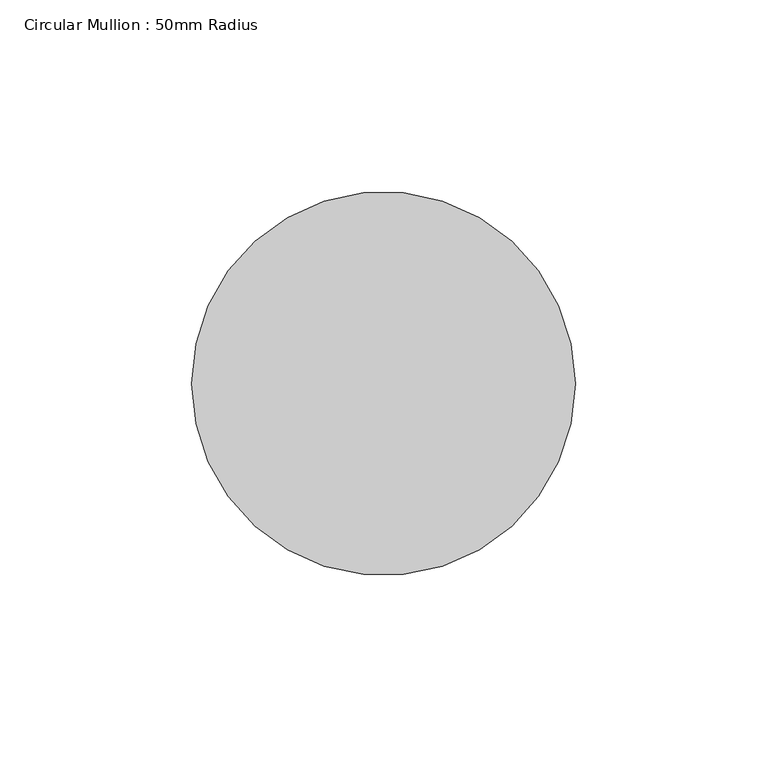
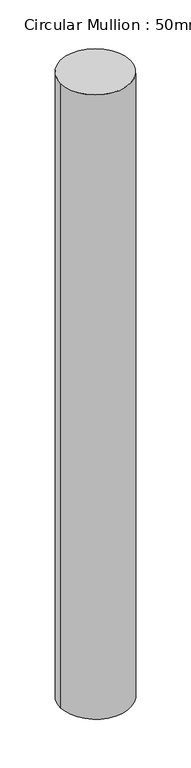
"""IFC4 building model written with IfcOpenShell, lengths in millimetres: member geometry, Circular Mullion : 50mm Radius."""

from ifc_helpers import new_model, si_unit, point, frame, origin, origin_2d, place, context, project, spatial, circle_curve, trimmed, segment, composite_curve, outline, extrude, source, transform, mapped, element, save


def circular_mullion_50mm_radius_0ba661d6(model_context):
    return source(origin(), model_context, "Body", "SweptSolid", [
        extrude(outline(composite_curve([segment(trimmed(circle_curve(origin_2d(), 50.0), [point((50.0, 0.0))], [point((-50.0, 0.0))], False, "CARTESIAN"), True, "CONTINUOUS"), segment(trimmed(circle_curve(origin_2d(), 50.0), [point((-50.0, 0.0))], [point((50.0, 0.0))], False, "CARTESIAN"), True, "CONTINUOUS")], self_intersect=False)), frame((0.0, 0.0, -945.5508716), z_axis=(0.0, 0.0, 1.0), x_axis=(1.0, 0.0, 0.0)), (0.0, 0.0, 1.0), 945.5508716),
    ])


if __name__ == "__main__":
    model = new_model("IFC4")
    model_context = context("Model", 3, world=origin())
    ifc_project = project(units=[si_unit("LENGTHUNIT", "METRE", prefix="MILLI")], contexts=[model_context])
    site = spatial("IfcSite", under=ifc_project)
    building = spatial("IfcBuilding", under=site)
    placement = place(None, origin())
    circular_mullion_50mm_radius_shape = circular_mullion_50mm_radius_0ba661d6(model_context)
    element("IfcMember", 1, ObjectType="Circular Mullion : 50mm Radius", at=placement, inside=building, context=model_context, shape_type="MappedRepresentation", body=[
        mapped(circular_mullion_50mm_radius_shape, transform((0.0, 0.0, 0.0), x_axis=(1.0, 0.0, 0.0), y_axis=(0.0, 1.0, 0.0), z_axis=(0.0, 0.0, 1.0))),
    ])
    save(model, "model.ifc")

# Revit data of these elements
# Type "Circular Mullion : 50mm Radius"
#   built-in parameter 1007350 = 0.164042 (stored number, unit not read)
# Element 1 (IfcMember, "Circular Mullion : 50mm Radius")
#   Materials on its faces: "Aluminium"
# Materials
#   "Aluminium": class "Metal", colour RGB 247 247 247, transparency 0, Description = "Aluminium 6061", Cost = 0
